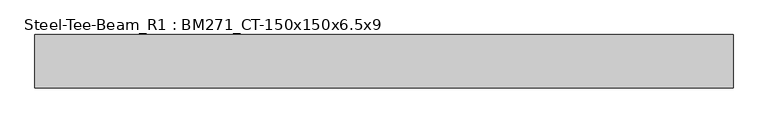
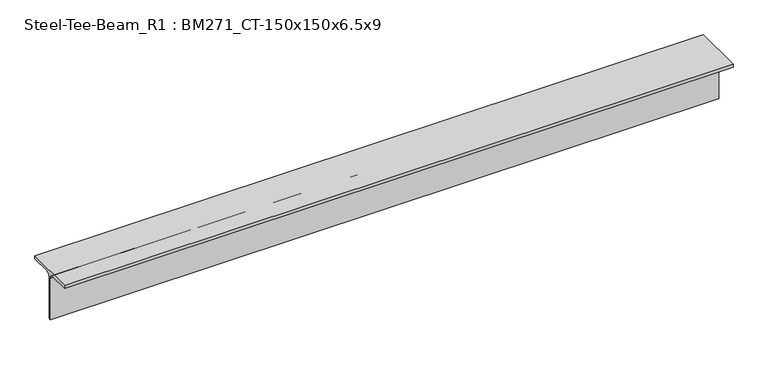
"""IFC4 building model written with IfcOpenShell, lengths in millimetres: member geometry, Steel-Tee-Beam_R1 : BM271_CT-150x150x6.5x9."""

from ifc_helpers import new_model, si_unit, point, frame, frame_2d, origin, place, context, project, spatial, polyline, circle_curve, trimmed, segment, composite_curve, outline, extrude, source, transform, mapped, element, save


def steel_tee_beam_r1_bm271_ct_150x150x6_5x9_7cb367b2(model_context):
    return source(origin(), model_context, "Body", "SweptSolid", [
        extrude(outline(composite_curve([segment(polyline([(-75.0, 75.0), (75.0, 75.0), (75.0, 66.0), (16.25, 66.0)]), True, "CONTINUOUS"), segment(trimmed(circle_curve(frame_2d((16.25, 53.0)), 13.0), [point((16.25, 66.0))], [point((3.25, 53.0))], True, "CARTESIAN"), True, "CONTINUOUS"), segment(polyline([(3.25, 53.0), (3.25, -75.0), (-3.25, -75.0), (-3.25, 53.0)]), True, "CONTINUOUS"), segment(trimmed(circle_curve(frame_2d((-16.25, 53.0)), 13.0), [point((-3.25, 53.0))], [point((-16.25, 66.0))], True, "CARTESIAN"), True, "CONTINUOUS"), segment(polyline([(-16.25, 66.0), (-75.0, 66.0), (-75.0, 75.0)]), True, "CONTINUOUS")], self_intersect=False)), frame((-1113.6541462, 0.0, 0.0), z_axis=(1.0, 0.0, 0.0), x_axis=(0.0, 1.0, 0.0)), (0.0, 0.0, 1.0), 1955.9770441),
    ])


if __name__ == "__main__":
    model = new_model("IFC4")
    model_context = context("Model", 3, world=origin())
    ifc_project = project(units=[si_unit("LENGTHUNIT", "METRE", prefix="MILLI")], contexts=[model_context])
    site = spatial("IfcSite", under=ifc_project)
    building = spatial("IfcBuilding", under=site)
    placement = place(None, origin())
    steel_tee_beam_r1_bm271_ct_150x150x6_5x9_shape = steel_tee_beam_r1_bm271_ct_150x150x6_5x9_7cb367b2(model_context)
    element("IfcMember", 1, ObjectType="Steel-Tee-Beam_R1 : BM271_CT-150x150x6.5x9", at=placement, inside=building, context=model_context, shape_type="MappedRepresentation", body=[
        mapped(steel_tee_beam_r1_bm271_ct_150x150x6_5x9_shape, transform((0.0, 0.0, 0.0), x_axis=(1.0, 0.0, 0.0), y_axis=(0.0, 1.0, 0.0), z_axis=(0.0, 0.0, 1.0))),
    ])
    save(model, "model.ifc")

# Revit data of these elements
# Type "Steel-Tee-Beam_R1 : BM271_CT-150x150x6.5x9"
#   Keynote = "CT-150x150x6.5x9"
#   Surface Area = 0.588841 m²/m
#   Section Area = 23.3904 cm²
#   Mass per Unit Length = 18.3614 kg/m
#   Length [instance default] = 1.5240 m
#   bf = 0.1500 m
#   d = 0.1500 m
#   k = 0.0220 m
#   r = 0.0130 m
#   tf = 0.0090 m
#   tw = 0.0065 m
#   hec_material4 [instance default] = none
#   hec_material3 [instance default] = none
#   hec_material2 [instance default] = none
#   hec_material1 [instance default] = none
#   Structural Material [instance default] = Steel, 45-345
#   Assembly Code = ""
# Element 1 (IfcMember, "Steel-Tee-Beam_R1 : BM271_CT-150x150x6.5x9")
#   Structural Material = none
# Materials
#   "Steel, 45-345": class "Metal", colour RGB 189 187 185, transparency 0, Description = "Steel 345 MPa", Cost = 0
